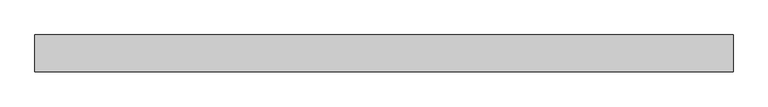
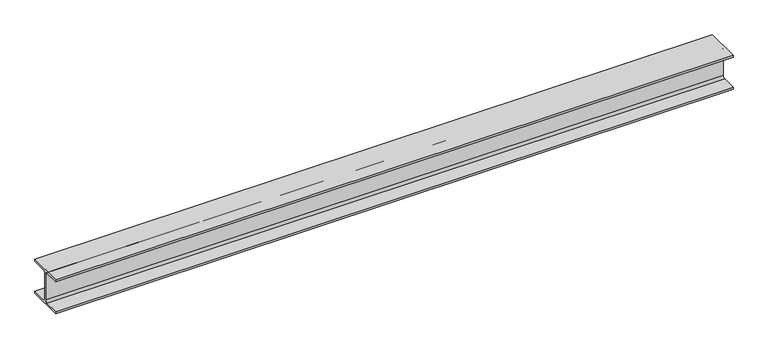
"""IFC4 building model written with IfcOpenShell, lengths in millimetres: beam geometry, 0912_Steel Framing_H-KSD3502 : H_SB_ASB_H-200x200x8x12."""

from ifc_helpers import new_model, si_unit, point, frame, frame_2d, origin, place, context, project, spatial, polyline, circle_curve, trimmed, segment, composite_curve, outline, extrude, source, transform, mapped, element, save


def beam_f40cded9(model_context):
    return source(origin(), model_context, "Body", "SweptSolid", [
        extrude(outline(composite_curve([segment(polyline([(100.0, -88.0), (100.0, -100.0), (-100.0, -100.0), (-100.0, -88.0), (-17.0, -88.0)]), True, "CONTINUOUS"), segment(trimmed(circle_curve(frame_2d((-17.0, -75.0)), 13.0), [point((-17.0, -88.0))], [point((-4.0, -75.0))], True, "CARTESIAN"), True, "CONTINUOUS"), segment(polyline([(-4.0, -75.0), (-4.0, 75.0)]), True, "CONTINUOUS"), segment(trimmed(circle_curve(frame_2d((-17.0, 75.0)), 13.0), [point((-4.0, 75.0))], [point((-17.0, 88.0))], True, "CARTESIAN"), True, "CONTINUOUS"), segment(polyline([(-17.0, 88.0), (-100.0, 88.0), (-100.0, 100.0), (100.0, 100.0), (100.0, 88.0), (17.0, 88.0)]), True, "CONTINUOUS"), segment(trimmed(circle_curve(frame_2d((17.0, 75.0)), 13.0), [point((17.0, 88.0))], [point((4.0, 75.0))], True, "CARTESIAN"), True, "CONTINUOUS"), segment(polyline([(4.0, 75.0), (4.0, -75.0)]), True, "CONTINUOUS"), segment(trimmed(circle_curve(frame_2d((17.0, -75.0)), 13.0), [point((4.0, -75.0))], [point((17.0, -88.0))], True, "CARTESIAN"), True, "CONTINUOUS"), segment(polyline([(17.0, -88.0), (100.0, -88.0)]), True, "CONTINUOUS")], self_intersect=False)), frame((-1951.6160937, 0.0, 0.0), z_axis=(1.0, 0.0, 0.0), x_axis=(0.0, 1.0, 0.0)), (0.0, 0.0, 1.0), 3785.2806295),
    ])


if __name__ == "__main__":
    model = new_model("IFC4")
    model_context = context("Model", 3, world=origin())
    ifc_project = project(units=[si_unit("LENGTHUNIT", "METRE", prefix="MILLI")], contexts=[model_context])
    site = spatial("IfcSite", under=ifc_project)
    building = spatial("IfcBuilding", under=site)
    placement = place(None, origin())
    beam_shape = beam_f40cded9(model_context)
    element("IfcBeam", 1, ObjectType="0912_Steel Framing_H-KSD3502 : H_SB_ASB_H-200x200x8x12", at=placement, inside=building, context=model_context, shape_type="MappedRepresentation", body=[
        mapped(beam_shape, transform((0.0, 0.0, 0.0), x_axis=(1.0, 0.0, 0.0), y_axis=(0.0, 1.0, 0.0), z_axis=(0.0, 0.0, 1.0))),
    ])
    save(model, "model.ifc")

# Revit data of these elements
# Type "0912_Steel Framing_H-KSD3502 : H_SB_ASB_H-200x200x8x12"
#   H_WM Code_1 = "S01AA002-00001 | Main Steel Structure Fabrication Work | Shelter/Building | Medium Steel - Standard (90KG/M>Weight≥30KG/M) | Material: (   )"
#   H_WM Code_2 = "S03AA028-00001 | Main Steel Structure Erection Work | Shelter/Building | Medium Steel (90KG/M>Weight≥30KG/M) | Material: (   )"
#   H_WM Code_3 = "S01AA010-00001 | Main Steel Structure Fabrication Work | Shelter/Building | Steel Painting/Coating | for Non-Fireproofed Steel Surface, Surface Preparation, Primer, Second & Final Coat | Material: (   )"
#   H_Q'ty Cal Type Tag = "SB-Q2"
#   Width = 20.0 cm
#   Web Thickness = 0.8 cm
#   Web Fillet = 1.3 cm
#   Warping Constant = 141000.0 cm⁶
#   W = 0
#   Torsional Moment of Inertia = 26.2485 cm⁴
#   Section Area = 63.53 cm²
#   Plastic Modulus weak axis = 244.0 cm³
#   Plastic Modulus strong axis = 525.0 cm³
#   Perimeter = 1.16 m²/m
#   Nominal Weight = 49.90 kgf/m
#   Moment of Inertia weak axis = 1600.00 cm⁴
#   Moment of Inertia strong axis = 4720.00 cm⁴
#   Height = 20.0 cm
#   Flange Thickness = 1.2 cm
#   Elastic Modulus weak axis = 160.0 cm³
#   Elastic Modulus strong axis = 472.0 cm³
#   Centroid Vertical = 10.0 cm
#   Centroid Horizontal = 10.0 cm
#   Ix = 47200000
#   Length [instance default] = 1.5240 m
#   Zx = 525000
#   b = 0.2000 m
#   h = 0.2000 m
#   r = 0.0130 m
#   s = 0.0080 m
#   t = 0.0120 m
#   A = 0.006353 m²
#   Structural Material [instance default] = Steel, 45-345
#   Assembly Code = ""
# Element 1 (IfcBeam, "0912_Steel Framing_H-KSD3502 : H_SB_ASB_H-200x200x8x12")
#   Structural Material = none
# Materials
#   "Steel, 45-345": class "Metal", colour RGB 189 187 185, transparency 0, Description = "Steel 345 MPa", Cost = 0
